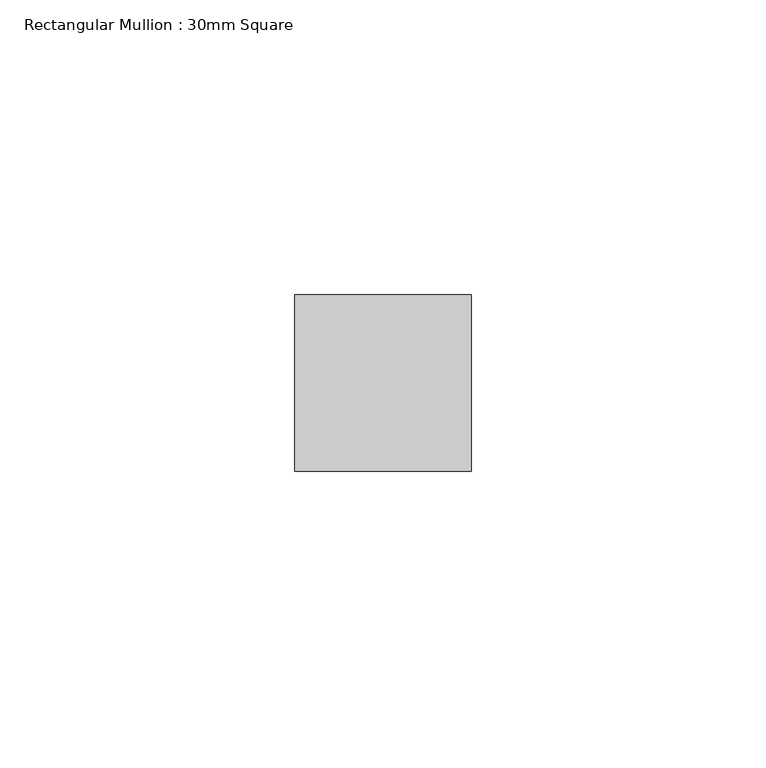
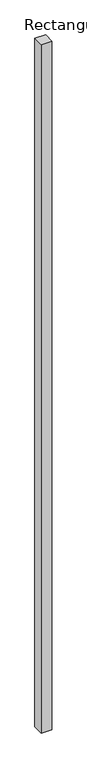
"""IFC4 building model written with IfcOpenShell, lengths in millimetres: member geometry, Rectangular Mullion : 30mm Square."""

from ifc_helpers import new_model, si_unit, frame, origin, place, context, project, spatial, polyline, outline, extrude, source, transform, mapped, element, save


def rectangular_mullion_30mm_square_c1d86b1d(model_context):
    return source(origin(), model_context, "Body", "SweptSolid", [
        extrude(outline(polyline([(15.0, 15.0), (15.0, -15.0), (-15.0, -15.0), (-15.0, 15.0), (15.0, 15.0)])), frame((0.0, 0.0, -2036.7851817), z_axis=(0.0, 0.0, 1.0), x_axis=(1.0, 0.0, 0.0)), (0.0, 0.0, 1.0), 2036.7851817),
    ])


if __name__ == "__main__":
    model = new_model("IFC4")
    model_context = context("Model", 3, world=origin())
    ifc_project = project(units=[si_unit("LENGTHUNIT", "METRE", prefix="MILLI")], contexts=[model_context])
    site = spatial("IfcSite", under=ifc_project)
    building = spatial("IfcBuilding", under=site)
    placement = place(None, origin())
    rectangular_mullion_30mm_square_shape = rectangular_mullion_30mm_square_c1d86b1d(model_context)
    element("IfcMember", 1, ObjectType="Rectangular Mullion : 30mm Square", at=placement, inside=building, context=model_context, shape_type="MappedRepresentation", body=[
        mapped(rectangular_mullion_30mm_square_shape, transform((0.0, 0.0, 0.0), x_axis=(1.0, 0.0, 0.0), y_axis=(0.0, 1.0, 0.0), z_axis=(0.0, 0.0, 1.0))),
    ])
    save(model, "model.ifc")

# Revit data of these elements
# Type "Rectangular Mullion : 30mm Square"
#   built-in parameter 1007304 = 0.0984252 (stored number, unit not read)
#   built-in parameter 1007301 = 0.0492126 (stored number, unit not read)
#   built-in parameter 1007300 = 0.0492126 (stored number, unit not read)
# Element 1 (IfcMember, "Rectangular Mullion : 30mm Square")
#   Materials on its faces: "Aluminum"
# Materials
#   "Aluminum": class "Metal", colour RGB 244 244 244, transparency 0, Description = "Aluminum 6061", Cost = 0
